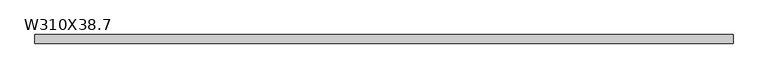
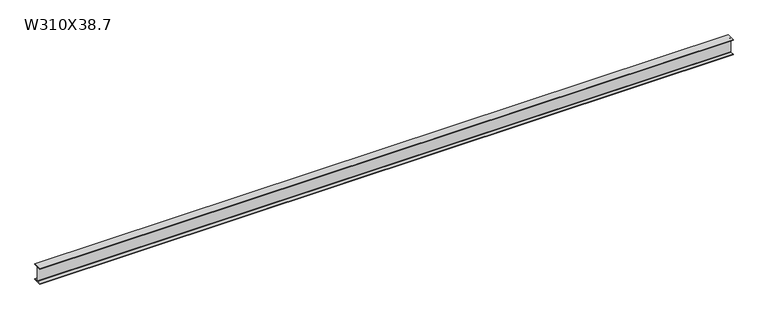
"""IFC4 building model written with IfcOpenShell, lengths in millimetres: beam geometry, M_W Shapes : W310X38.7."""

from ifc_helpers import new_model, si_unit, point, frame, frame_2d, origin, place, context, project, spatial, polyline, circle_curve, trimmed, segment, composite_curve, outline, extrude, source, transform, mapped, element, save


def w310x38_7_4aa3e629(model_context):
    return source(origin(), model_context, "Body", "SweptSolid", [
        extrude(outline(composite_curve([segment(polyline([(82.5, -145.35), (82.5, -155.0), (-82.5, -155.0), (-82.5, -145.35), (-10.57, -145.35)]), True, "CONTINUOUS"), segment(trimmed(circle_curve(frame_2d((-10.57, -137.7)), 7.65), [point((-10.57, -145.35))], [point((-2.92, -137.7))], True, "CARTESIAN"), True, "CONTINUOUS"), segment(polyline([(-2.92, -137.7), (-2.92, 137.7)]), True, "CONTINUOUS"), segment(trimmed(circle_curve(frame_2d((-10.57, 137.7)), 7.65), [point((-2.92, 137.7))], [point((-10.57, 145.35))], True, "CARTESIAN"), True, "CONTINUOUS"), segment(polyline([(-10.57, 145.35), (-82.5, 145.35), (-82.5, 155.0), (82.5, 155.0), (82.5, 145.35), (10.57, 145.35)]), True, "CONTINUOUS"), segment(trimmed(circle_curve(frame_2d((10.57, 137.7)), 7.65), [point((10.57, 145.35))], [point((2.92, 137.7))], True, "CARTESIAN"), True, "CONTINUOUS"), segment(polyline([(2.92, 137.7), (2.92, -137.7)]), True, "CONTINUOUS"), segment(trimmed(circle_curve(frame_2d((10.57, -137.7)), 7.65), [point((2.92, -137.7))], [point((10.57, -145.35))], True, "CARTESIAN"), True, "CONTINUOUS"), segment(polyline([(10.57, -145.35), (82.5, -145.35)]), True, "CONTINUOUS")], self_intersect=False)), frame((-6518.15, 0.0, 0.0), z_axis=(1.0, 0.0, 0.0), x_axis=(0.0, 1.0, 0.0)), (0.0, 0.0, 1.0), 13402.4),
    ])


if __name__ == "__main__":
    model = new_model("IFC4")
    model_context = context("Model", 3, world=origin())
    ifc_project = project(units=[si_unit("LENGTHUNIT", "METRE", prefix="MILLI")], contexts=[model_context])
    site = spatial("IfcSite", under=ifc_project)
    building = spatial("IfcBuilding", under=site)
    placement = place(None, origin())
    w310x38_7_shape = w310x38_7_4aa3e629(model_context)
    element("IfcBeam", 1, ObjectType="M_W Shapes : W310X38.7", at=placement, inside=building, context=model_context, shape_type="MappedRepresentation", body=[
        mapped(w310x38_7_shape, transform((0.0, 0.0, 0.0), x_axis=(1.0, 0.0, 0.0), y_axis=(0.0, 1.0, 0.0), z_axis=(0.0, 0.0, 1.0))),
    ])
    save(model, "model.ifc")

# Revit data of these elements
# Type "M_W Shapes : W310X38.7"
#   Section Name Key = "W12x26"
#   Width = 165 mm
#   Web Thickness = 5.84 mm
#   Web Fillet = 7.65 mm
#   Warping Constant = 163000 cm⁶
#   Torsional Moment of Inertia = 12.5 cm⁴
#   Section Area = 49.4 cm²
#   Plastic Modulus weak axis = 0.00473217 (stored number, unit not read)
#   Plastic Modulus strong axis = 0.0215419 (stored number, unit not read)
#   Perimeter = 1.25 m²/m
#   Nominal Weight = 379.516 N/m
#   Moment of Inertia weak axis = 720 cm⁴
#   Moment of Inertia strong axis = 8490 cm⁴
#   Height = 310 mm
#   Flange Thickness = 9.65 mm
#   Elastic Modulus weak axis = 0.00309003 (stored number, unit not read)
#   Elastic Modulus strong axis = 0.0193171 (stored number, unit not read)
#   Centroid Vertical = 155 mm
#   Centroid Horizontal = 82.5 mm
#   Length [instance default] = 1.5 m
#   Structural Material [instance default] = Steel, 45-345
#   Assembly Code = ""
# Element 1 (IfcBeam, "M_W Shapes : W310X38.7")
#   Materials on its faces: "Steel, 45-345"
# Materials
#   "Steel, 45-345": class "Metal", colour RGB 189 187 185, transparency 0, Description = "Steel 345 MPa", Cost = 0
